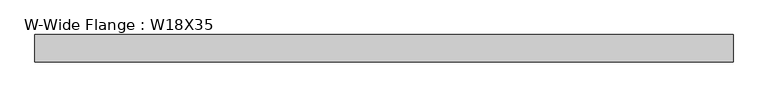
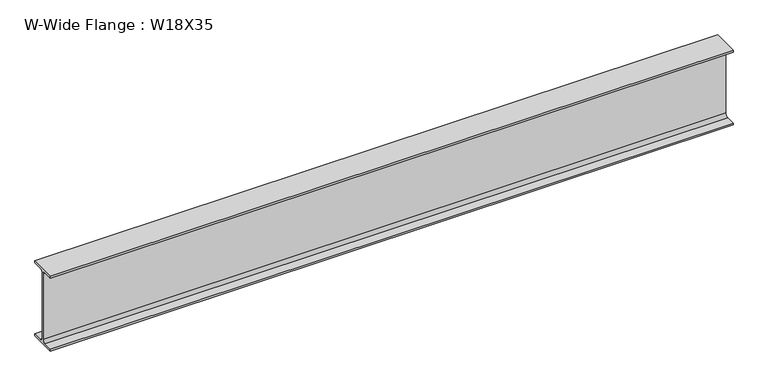
"""IFC4 building model written with IfcOpenShell, lengths in millimetres: beam geometry, W-Wide Flange : W18X35."""

import ifcopenshell
import ifcopenshell.guid

model = None  # the IFC model being written
_history = None  # IfcOwnerHistory: only IFC2X3 demands one
_inside = {}  # id of a spatial element -> (the spatial element, [elements in it])
_under = {}  # id of a project, library or spatial element -> (it, [spatial elements below it])
_declared = {}  # id of a project -> (the project, [libraries it declares])
_typed = {}  # id of a type object -> (the type object, [elements of that type])
_made_of = {}  # id of a material, layer set ... -> (it, [elements and type objects made of it])


def new_model(schema):
    """Start an empty IFC model of exactly this schema.

    Asked for "IFC4X3", IfcOpenShell would pick the latest addendum, in which some entities
    have other attributes; the version numbers below select the first issue.
    IFC2X3 requires an IfcOwnerHistory on every rooted entity: one is made here for all.
    """
    global model, _history
    if schema == "IFC4X3":
        model = ifcopenshell.file(schema_version=(4, 3, 0, 0))
    else:
        model = ifcopenshell.file(schema=schema)
    _inside.clear()
    _under.clear()
    _declared.clear()
    _typed.clear()
    _made_of.clear()
    _history = None
    if model.schema == "IFC2X3":
        org = make("IfcOrganization", Name="unknown")
        user = make(
            "IfcPersonAndOrganization",
            ThePerson=make("IfcPerson", FamilyName="unknown"),
            TheOrganization=org,
        )
        app = make(
            "IfcApplication",
            ApplicationDeveloper=org,
            Version="unknown",
            ApplicationFullName="unknown",
            ApplicationIdentifier="unknown",
        )
        _history = make(
            "IfcOwnerHistory",
            OwningUser=user,
            OwningApplication=app,
            ChangeAction="ADDED",
            CreationDate=0,
        )
    return model


def make(cls, **values):
    """One entity of the class cls with the attributes given. An attribute that is None is left unset."""
    return model.create_entity(
        cls, **{name: value for name, value in values.items() if value is not None}
    )


def rooted(cls, **values):
    """An entity with a GlobalId (a new one), such as an element, a storey or a relation."""
    return make(cls, GlobalId=ifcopenshell.guid.new(), OwnerHistory=_history, **values)


def si_unit(unit_type, name, prefix=None):
    """IfcSIUnit, for example si_unit("LENGTHUNIT", "METRE", prefix="MILLI")."""
    return make("IfcSIUnit", UnitType=unit_type, Prefix=prefix, Name=name)


def assignment(units):
    """IfcUnitAssignment: the units of a project."""
    return None if units is None else make("IfcUnitAssignment", Units=units)


def point(xyz):
    """IfcCartesianPoint."""
    return None if xyz is None else make("IfcCartesianPoint", Coordinates=xyz)


def direction(xyz):
    """IfcDirection."""
    return None if xyz is None else make("IfcDirection", DirectionRatios=xyz)


def frame(location, z_axis=None, x_axis=None):
    """IfcAxis2Placement3D, a coordinate frame: its origin and axes. An axis left out is left unset."""
    return make(
        "IfcAxis2Placement3D",
        Location=point(location),
        Axis=direction(z_axis),
        RefDirection=direction(x_axis),
    )


def frame_2d(location, x_axis=None):
    """IfcAxis2Placement2D, a coordinate frame in the plane: its origin and x axis."""
    return make(
        "IfcAxis2Placement2D", Location=point(location), RefDirection=direction(x_axis)
    )


def origin():
    """The frame at (0, 0, 0) with its axes left unset."""
    return frame((0.0, 0.0, 0.0))


def place(relative_to, where):
    """IfcLocalPlacement: puts the frame where relative to a parent placement (None: the world)."""
    return make(
        "IfcLocalPlacement", PlacementRelTo=relative_to, RelativePlacement=where
    )


def context(
    kind, dimensions, precision=None, world=None, true_north=None, identifier=None
):
    """IfcGeometricRepresentationContext, for example the 3D "Model" context."""
    return make(
        "IfcGeometricRepresentationContext",
        ContextIdentifier=identifier,
        ContextType=kind,
        CoordinateSpaceDimension=dimensions,
        Precision=precision,
        WorldCoordinateSystem=world,
        TrueNorth=true_north,
    )


def project(units=None, contexts=None):
    """IfcProject with its units and contexts."""
    return rooted(
        "IfcProject",
        Name="project",
        RepresentationContexts=contexts,
        UnitsInContext=assignment(units),
    )


def spatial(cls, under=None, at=None, **own):
    """A site, building, storey or space (cls), placed at a placement, below another one or the project."""
    s = rooted(cls, ObjectPlacement=at, **own)
    if under is not None:
        _under.setdefault(under.id(), (under, []))[1].append(s)
    return s


def polyline(points):
    """IfcPolyline through the points."""
    return make("IfcPolyline", Points=[point(p) for p in points])


def circle_curve(where, radius):
    """IfcCircle in the frame where."""
    return make("IfcCircle", Position=where, Radius=radius)


def trimmed(basis, trim1, trim2, sense, master):
    """IfcTrimmedCurve: the piece of a basis curve between two trims."""
    return make(
        "IfcTrimmedCurve",
        BasisCurve=basis,
        Trim1=trim1,
        Trim2=trim2,
        SenseAgreement=sense,
        MasterRepresentation=master,
    )


def segment(curve, same_sense, transition):
    """IfcCompositeCurveSegment."""
    return make(
        "IfcCompositeCurveSegment",
        Transition=transition,
        SameSense=same_sense,
        ParentCurve=curve,
    )


def composite_curve(segments, self_intersect=None):
    """IfcCompositeCurve: segments joined end to end."""
    return make("IfcCompositeCurve", Segments=segments, SelfIntersect=self_intersect)


def outline(outer, holes=None, kind="AREA"):
    """IfcArbitraryClosedProfileDef: a profile drawn as a closed curve; with holes, ...WithVoids."""
    if holes is None:
        return make("IfcArbitraryClosedProfileDef", ProfileType=kind, OuterCurve=outer)
    return make(
        "IfcArbitraryProfileDefWithVoids",
        ProfileType=kind,
        OuterCurve=outer,
        InnerCurves=holes,
    )


def extrude(swept, where, along, depth):
    """IfcExtrudedAreaSolid: the profile swept, set in the frame where, extruded along a direction by depth."""
    return make(
        "IfcExtrudedAreaSolid",
        SweptArea=swept,
        Position=where,
        ExtrudedDirection=direction(along),
        Depth=depth,
    )


def shape(context_of_items, identifier, shape_type, items):
    """IfcShapeRepresentation: the items that make up one representation, for example the "Body"."""
    return make(
        "IfcShapeRepresentation",
        ContextOfItems=context_of_items,
        RepresentationIdentifier=identifier,
        RepresentationType=shape_type,
        Items=items,
    )


def source(mapping_origin, context_of_items, identifier, shape_type, items):
    """IfcRepresentationMap: a shape defined once, which mapped items show again and again."""
    return make(
        "IfcRepresentationMap",
        MappingOrigin=mapping_origin,
        MappedRepresentation=shape(context_of_items, identifier, shape_type, items),
    )


def transform(
    local_origin,
    x_axis=None,
    y_axis=None,
    z_axis=None,
    scale=None,
    scale2=None,
    scale3=None,
    uniform=True,
):
    """IfcCartesianTransformationOperator3D, or its non-uniform kind. x_axis, y_axis, z_axis: its Axis1, 2, 3."""
    if uniform:
        return make(
            "IfcCartesianTransformationOperator3D",
            Axis1=direction(x_axis),
            Axis2=direction(y_axis),
            LocalOrigin=point(local_origin),
            Scale=scale,
            Axis3=direction(z_axis),
        )
    return make(
        "IfcCartesianTransformationOperator3DnonUniform",
        Axis1=direction(x_axis),
        Axis2=direction(y_axis),
        LocalOrigin=point(local_origin),
        Scale=scale,
        Axis3=direction(z_axis),
        Scale2=scale2,
        Scale3=scale3,
    )


def mapped(mapping_source, mapping_target):
    """IfcMappedItem: shows the shape of a source again, moved by a transform."""
    return make(
        "IfcMappedItem", MappingSource=mapping_source, MappingTarget=mapping_target
    )


def made_of(thing, what):
    """Note that an element or type object is made of a material, layer set ...; save() writes the relation."""
    if what is not None:
        _made_of.setdefault(what.id(), (what, []))[1].append(thing)
    return thing


def element(
    cls,
    number,
    at=None,
    inside=None,
    cuts=None,
    type_object=None,
    material=None,
    context=None,
    identifier="Body",
    shape_type=None,
    held_by="IfcProductDefinitionShape",
    body=None,
    shapes=None,
    **own,
):
    """One element of the class cls, such as IfcWall. Its Tag is "e" and its number.

    at: its placement. inside: the storey or other place that contains it. cuts: it is an
    opening in that element (IfcRelVoidsElement). A single representation is given by context,
    identifier, shape_type and body (its items); several are given by shapes. held_by: the class
    of the entity that holds the representations. save() writes the other relations.
    """
    e = rooted(cls, Tag="e%d" % number, ObjectPlacement=at, **own)
    if body is not None:
        shapes = [shape(context, identifier, shape_type, body)]
    if shapes is not None:
        e.Representation = make(held_by, Representations=shapes)
    if inside is not None:
        _inside.setdefault(inside.id(), (inside, []))[1].append(e)
    if cuts is not None:
        rooted(
            "IfcRelVoidsElement", RelatingBuildingElement=cuts, RelatedOpeningElement=e
        )
    if type_object is not None:
        _typed.setdefault(type_object.id(), (type_object, []))[1].append(e)
    return made_of(e, material)


def aggregate(whole, parts):
    """IfcRelAggregates: a whole, such as a stair, and the parts it consists of."""
    return rooted("IfcRelAggregates", RelatingObject=whole, RelatedObjects=parts)


def save(model, path):
    """Write the relations noted so far, then the file.

    IfcRelAggregates (storeys below a building ...), IfcRelContainedInSpatialStructure (elements
    in a storey), IfcRelDefinesByType, IfcRelAssociatesMaterial and IfcRelDeclares: one each for
    every whole, place, type object, material and project.
    """
    for whole, parts in _under.values():
        aggregate(whole, parts)
    for where, things in _inside.values():
        rooted(
            "IfcRelContainedInSpatialStructure",
            RelatedElements=things,
            RelatingStructure=where,
        )
    for kind, things in _typed.values():
        rooted("IfcRelDefinesByType", RelatedObjects=things, RelatingType=kind)
    for what, things in _made_of.values():
        rooted("IfcRelAssociatesMaterial", RelatedObjects=things, RelatingMaterial=what)
    for by, libraries in _declared.values():
        rooted("IfcRelDeclares", RelatingContext=by, RelatedDefinitions=libraries)
    model.write(path)


def w_wide_flange_w18x35_53c17956(model_context):
    return source(origin(), model_context, "Body", "SweptSolid", [
        extrude(outline(composite_curve([segment(polyline([(76.2, -213.995), (76.2, -224.79), (-76.2, -224.79), (-76.2, -213.995), (-21.59, -213.995)]), True, "CONTINUOUS"), segment(trimmed(circle_curve(frame_2d((-21.59, -196.215)), 17.78), [point((-21.59, -213.995))], [point((-3.81, -196.215))], True, "CARTESIAN"), True, "CONTINUOUS"), segment(polyline([(-3.81, -196.215), (-3.81, 196.215)]), True, "CONTINUOUS"), segment(trimmed(circle_curve(frame_2d((-21.59, 196.215)), 17.78), [point((-3.81, 196.215))], [point((-21.59, 213.995))], True, "CARTESIAN"), True, "CONTINUOUS"), segment(polyline([(-21.59, 213.995), (-76.2, 213.995), (-76.2, 224.79), (76.2, 224.79), (76.2, 213.995), (21.59, 213.995)]), True, "CONTINUOUS"), segment(trimmed(circle_curve(frame_2d((21.59, 196.215)), 17.78), [point((21.59, 213.995))], [point((3.81, 196.215))], True, "CARTESIAN"), True, "CONTINUOUS"), segment(polyline([(3.81, 196.215), (3.81, -196.215)]), True, "CONTINUOUS"), segment(trimmed(circle_curve(frame_2d((21.59, -196.215)), 17.78), [point((3.81, -196.215))], [point((21.59, -213.995))], True, "CARTESIAN"), True, "CONTINUOUS"), segment(polyline([(21.59, -213.995), (76.2, -213.995)]), True, "CONTINUOUS")], self_intersect=False)), frame((-1943.1, 0.0, 0.0), z_axis=(1.0, 0.0, 0.0), x_axis=(0.0, 1.0, 0.0)), (0.0, 0.0, 1.0), 3886.2),
    ])


if __name__ == "__main__":
    model = new_model("IFC4")
    model_context = context("Model", 3, world=origin())
    ifc_project = project(units=[si_unit("LENGTHUNIT", "METRE", prefix="MILLI")], contexts=[model_context])
    site = spatial("IfcSite", under=ifc_project)
    building = spatial("IfcBuilding", under=site)
    placement = place(None, origin())
    w_wide_flange_w18x35_shape = w_wide_flange_w18x35_53c17956(model_context)
    element("IfcBeam", 1, ObjectType="W-Wide Flange : W18X35", at=placement, inside=building, context=model_context, shape_type="MappedRepresentation", body=[
        mapped(w_wide_flange_w18x35_shape, transform((0.0, 0.0, 0.0), x_axis=(1.0, 0.0, 0.0), y_axis=(0.0, 1.0, 0.0), z_axis=(0.0, 0.0, 1.0))),
    ])
    save(model, "model.ifc")

# Revit data of these elements
# Type "W-Wide Flange : W18X35"
#   Assembly Code = "B10"
#   W = 35
#   Length [instance default] = 5' - 0"
#   bf = 0' - 6"
#   d = 1' - 5.7"
#   k = 0' - 1 1/8"
#   k2 = 0' - 0.7"
#   tf = 0' - 0.425"
#   tw = 0' - 0.3"
#   A = 0.0715278 SF
#   Structural Material [instance default] = Steel ASTM A992
# Element 1 (IfcBeam, "W-Wide Flange : W18X35")
#   Materials on its faces: "Steel ASTM A992"
# Materials
#   "Steel ASTM A992": class "Metal", colour RGB 199 199 199, transparency 0, Description = "Structural steel 50ksi", Cost = 0
